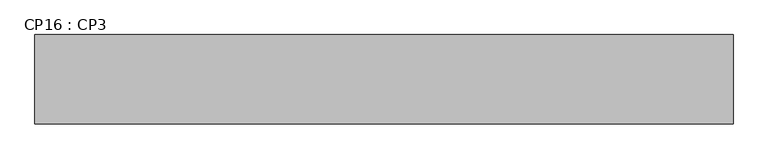
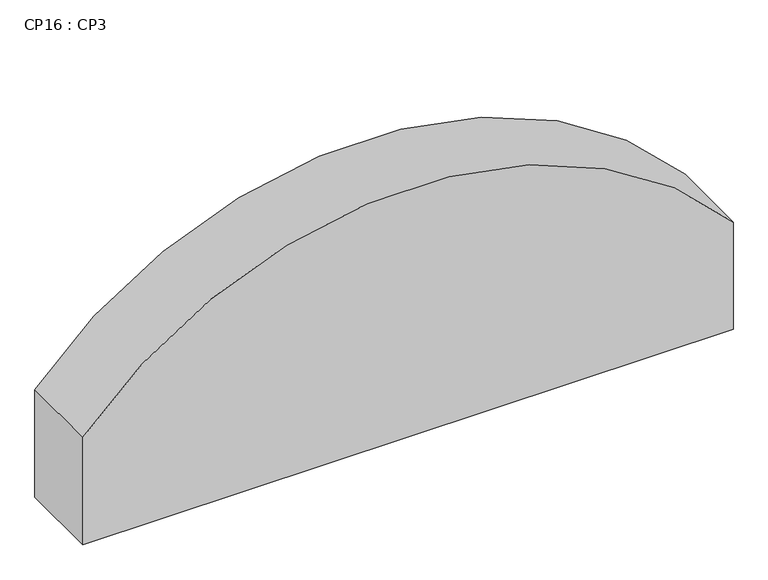
"""IFC4 building model written with IfcOpenShell, lengths in millimetres: beam geometry, CP16 : CP3."""

import ifcopenshell
import ifcopenshell.guid

model = None  # the IFC model being written
_history = None  # IfcOwnerHistory: only IFC2X3 demands one
_inside = {}  # id of a spatial element -> (the spatial element, [elements in it])
_under = {}  # id of a project, library or spatial element -> (it, [spatial elements below it])
_declared = {}  # id of a project -> (the project, [libraries it declares])
_typed = {}  # id of a type object -> (the type object, [elements of that type])
_made_of = {}  # id of a material, layer set ... -> (it, [elements and type objects made of it])


def new_model(schema):
    """Start an empty IFC model of exactly this schema.

    Asked for "IFC4X3", IfcOpenShell would pick the latest addendum, in which some entities
    have other attributes; the version numbers below select the first issue.
    IFC2X3 requires an IfcOwnerHistory on every rooted entity: one is made here for all.
    """
    global model, _history
    if schema == "IFC4X3":
        model = ifcopenshell.file(schema_version=(4, 3, 0, 0))
    else:
        model = ifcopenshell.file(schema=schema)
    _inside.clear()
    _under.clear()
    _declared.clear()
    _typed.clear()
    _made_of.clear()
    _history = None
    if model.schema == "IFC2X3":
        org = make("IfcOrganization", Name="unknown")
        user = make(
            "IfcPersonAndOrganization",
            ThePerson=make("IfcPerson", FamilyName="unknown"),
            TheOrganization=org,
        )
        app = make(
            "IfcApplication",
            ApplicationDeveloper=org,
            Version="unknown",
            ApplicationFullName="unknown",
            ApplicationIdentifier="unknown",
        )
        _history = make(
            "IfcOwnerHistory",
            OwningUser=user,
            OwningApplication=app,
            ChangeAction="ADDED",
            CreationDate=0,
        )
    return model


def make(cls, **values):
    """One entity of the class cls with the attributes given. An attribute that is None is left unset."""
    return model.create_entity(
        cls, **{name: value for name, value in values.items() if value is not None}
    )


def rooted(cls, **values):
    """An entity with a GlobalId (a new one), such as an element, a storey or a relation."""
    return make(cls, GlobalId=ifcopenshell.guid.new(), OwnerHistory=_history, **values)


def si_unit(unit_type, name, prefix=None):
    """IfcSIUnit, for example si_unit("LENGTHUNIT", "METRE", prefix="MILLI")."""
    return make("IfcSIUnit", UnitType=unit_type, Prefix=prefix, Name=name)


def assignment(units):
    """IfcUnitAssignment: the units of a project."""
    return None if units is None else make("IfcUnitAssignment", Units=units)


def point(xyz):
    """IfcCartesianPoint."""
    return None if xyz is None else make("IfcCartesianPoint", Coordinates=xyz)


def direction(xyz):
    """IfcDirection."""
    return None if xyz is None else make("IfcDirection", DirectionRatios=xyz)


def frame(location, z_axis=None, x_axis=None):
    """IfcAxis2Placement3D, a coordinate frame: its origin and axes. An axis left out is left unset."""
    return make(
        "IfcAxis2Placement3D",
        Location=point(location),
        Axis=direction(z_axis),
        RefDirection=direction(x_axis),
    )


def origin():
    """The frame at (0, 0, 0) with its axes left unset."""
    return frame((0.0, 0.0, 0.0))


def place(relative_to, where):
    """IfcLocalPlacement: puts the frame where relative to a parent placement (None: the world)."""
    return make(
        "IfcLocalPlacement", PlacementRelTo=relative_to, RelativePlacement=where
    )


def context(
    kind, dimensions, precision=None, world=None, true_north=None, identifier=None
):
    """IfcGeometricRepresentationContext, for example the 3D "Model" context."""
    return make(
        "IfcGeometricRepresentationContext",
        ContextIdentifier=identifier,
        ContextType=kind,
        CoordinateSpaceDimension=dimensions,
        Precision=precision,
        WorldCoordinateSystem=world,
        TrueNorth=true_north,
    )


def project(units=None, contexts=None):
    """IfcProject with its units and contexts."""
    return rooted(
        "IfcProject",
        Name="project",
        RepresentationContexts=contexts,
        UnitsInContext=assignment(units),
    )


def spatial(cls, under=None, at=None, **own):
    """A site, building, storey or space (cls), placed at a placement, below another one or the project."""
    s = rooted(cls, ObjectPlacement=at, **own)
    if under is not None:
        _under.setdefault(under.id(), (under, []))[1].append(s)
    return s


def circle_curve(where, radius):
    """IfcCircle in the frame where."""
    return make("IfcCircle", Position=where, Radius=radius)


def shape(context_of_items, identifier, shape_type, items):
    """IfcShapeRepresentation: the items that make up one representation, for example the "Body"."""
    return make(
        "IfcShapeRepresentation",
        ContextOfItems=context_of_items,
        RepresentationIdentifier=identifier,
        RepresentationType=shape_type,
        Items=items,
    )


def source(mapping_origin, context_of_items, identifier, shape_type, items):
    """IfcRepresentationMap: a shape defined once, which mapped items show again and again."""
    return make(
        "IfcRepresentationMap",
        MappingOrigin=mapping_origin,
        MappedRepresentation=shape(context_of_items, identifier, shape_type, items),
    )


def transform(
    local_origin,
    x_axis=None,
    y_axis=None,
    z_axis=None,
    scale=None,
    scale2=None,
    scale3=None,
    uniform=True,
):
    """IfcCartesianTransformationOperator3D, or its non-uniform kind. x_axis, y_axis, z_axis: its Axis1, 2, 3."""
    if uniform:
        return make(
            "IfcCartesianTransformationOperator3D",
            Axis1=direction(x_axis),
            Axis2=direction(y_axis),
            LocalOrigin=point(local_origin),
            Scale=scale,
            Axis3=direction(z_axis),
        )
    return make(
        "IfcCartesianTransformationOperator3DnonUniform",
        Axis1=direction(x_axis),
        Axis2=direction(y_axis),
        LocalOrigin=point(local_origin),
        Scale=scale,
        Axis3=direction(z_axis),
        Scale2=scale2,
        Scale3=scale3,
    )


def mapped(mapping_source, mapping_target):
    """IfcMappedItem: shows the shape of a source again, moved by a transform."""
    return make(
        "IfcMappedItem", MappingSource=mapping_source, MappingTarget=mapping_target
    )


def made_of(thing, what):
    """Note that an element or type object is made of a material, layer set ...; save() writes the relation."""
    if what is not None:
        _made_of.setdefault(what.id(), (what, []))[1].append(thing)
    return thing


def element(
    cls,
    number,
    at=None,
    inside=None,
    cuts=None,
    type_object=None,
    material=None,
    context=None,
    identifier="Body",
    shape_type=None,
    held_by="IfcProductDefinitionShape",
    body=None,
    shapes=None,
    **own,
):
    """One element of the class cls, such as IfcWall. Its Tag is "e" and its number.

    at: its placement. inside: the storey or other place that contains it. cuts: it is an
    opening in that element (IfcRelVoidsElement). A single representation is given by context,
    identifier, shape_type and body (its items); several are given by shapes. held_by: the class
    of the entity that holds the representations. save() writes the other relations.
    """
    e = rooted(cls, Tag="e%d" % number, ObjectPlacement=at, **own)
    if body is not None:
        shapes = [shape(context, identifier, shape_type, body)]
    if shapes is not None:
        e.Representation = make(held_by, Representations=shapes)
    if inside is not None:
        _inside.setdefault(inside.id(), (inside, []))[1].append(e)
    if cuts is not None:
        rooted(
            "IfcRelVoidsElement", RelatingBuildingElement=cuts, RelatedOpeningElement=e
        )
    if type_object is not None:
        _typed.setdefault(type_object.id(), (type_object, []))[1].append(e)
    return made_of(e, material)


def aggregate(whole, parts):
    """IfcRelAggregates: a whole, such as a stair, and the parts it consists of."""
    return rooted("IfcRelAggregates", RelatingObject=whole, RelatedObjects=parts)


def save(model, path):
    """Write the relations noted so far, then the file.

    IfcRelAggregates (storeys below a building ...), IfcRelContainedInSpatialStructure (elements
    in a storey), IfcRelDefinesByType, IfcRelAssociatesMaterial and IfcRelDeclares: one each for
    every whole, place, type object, material and project.
    """
    for whole, parts in _under.values():
        aggregate(whole, parts)
    for where, things in _inside.values():
        rooted(
            "IfcRelContainedInSpatialStructure",
            RelatedElements=things,
            RelatingStructure=where,
        )
    for kind, things in _typed.values():
        rooted("IfcRelDefinesByType", RelatedObjects=things, RelatingType=kind)
    for what, things in _made_of.values():
        rooted("IfcRelAssociatesMaterial", RelatedObjects=things, RelatingMaterial=what)
    for by, libraries in _declared.values():
        rooted("IfcRelDeclares", RelatingContext=by, RelatedDefinitions=libraries)
    model.write(path)


def plane_surface(at):
    """IfcPlane: the flat surface through the origin of the frame at, square to its z axis."""
    return make("IfcPlane", Position=at)


def cylinder_surface(at, radius):
    """IfcCylindricalSurface: all points at the distance radius from the z axis of the frame at."""
    return make("IfcCylindricalSurface", Position=at, Radius=radius)


def advanced_brep(points, edges, surfaces, faces):
    """IfcAdvancedBrep: a solid bounded by faces that lie on surfaces and meet in shared edges.

    An edge is (start, end): straight between two places in points (the first is 0);
    or (start, end, curve); or (start, end, curve, False) where it runs against its curve.
    A face is (place in surfaces, loops), or (place, loops, False) where it looks against
    its surface's normal. A loop lists edges by number (the first is 1), with a minus sign
    where the edge is run from its end to its start. The first loop is the outer one.
    """
    corners = [point(p) for p in points]
    vertices = [make("IfcVertexPoint", VertexGeometry=c) for c in corners]
    made = []
    for start, end, *more in edges:
        made.append(
            make(
                "IfcEdgeCurve",
                EdgeStart=vertices[start],
                EdgeEnd=vertices[end],
                EdgeGeometry=more[0] if more else make("IfcPolyline", Points=[corners[start], corners[end]]),
                SameSense=more[1] if len(more) > 1 else True,
            )
        )
    hull = []
    for where, loops, *sense in faces:
        bounds = []
        for j, loop in enumerate(loops):
            ring = [make("IfcOrientedEdge", EdgeElement=made[abs(k) - 1], Orientation=k > 0) for k in loop]
            bounds.append(
                make(
                    "IfcFaceOuterBound" if j == 0 else "IfcFaceBound",
                    Bound=make("IfcEdgeLoop", EdgeList=ring),
                    Orientation=True,
                )
            )
        hull.append(make("IfcAdvancedFace", Bounds=bounds, FaceSurface=surfaces[where], SameSense=sense[0] if sense else True))
    return make("IfcAdvancedBrep", Outer=make("IfcClosedShell", CfsFaces=hull))


def cp16_cp3_4619df2a(model_context):
    return source(origin(), model_context, "Body", "AdvancedBrep", [
        advanced_brep(
        [(10143.2245521, 20099.7448193, 13800.0), (10143.2245521, 20099.7448193, 14620.0), (14843.2245541, 20099.7448193, 14620.0), (14843.2245527, 20099.7448193, 13800.0), (14843.2245541, 19499.6999972, 14620.0), (10143.2245541, 19499.6999972, 14620.0), (10143.2245521, 19499.6999972, 13800.0), (14843.2245527, 19499.6999972, 13800.0)],
        [
            (0, 1),
            (1, 2, circle_curve(frame((12493.2245541, 20099.7448193, 12603.2870371), z_axis=(0.0, 1.0, 0.0), x_axis=(0.0, 0.0, -1.0)), 3096.7129629)),
            (2, 3),
            (3, 0),
            (4, 5, circle_curve(frame((12493.2245541, 19499.6999972, 12603.2870371), z_axis=(0.0, -1.0, 0.0), x_axis=(0.0, 0.0, -1.0)), 3096.7129629)),
            (5, 6),
            (6, 7),
            (7, 4),
            (6, 0),
            (3, 7),
            (4, 2),
            (1, 5),
        ],
        [
            plane_surface(frame((9993.2245542, 20099.7448193, 13800.0), z_axis=(0.0, 1.0, 0.0), x_axis=(0.0, 0.0, 1.0))),
            plane_surface(frame((9993.2245542, 19499.6999972, 13800.0), z_axis=(0.0, -1.0, 0.0), x_axis=(0.0, 0.0, -1.0))),
            plane_surface(frame((14993.2245542, 20099.7448193, 13800.0), z_axis=(0.0, 0.0, -1.0), x_axis=(0.0, -1.0, 0.0))),
            cylinder_surface(frame((12493.2245541, 20099.7448193, 12603.2870371), z_axis=(0.0, 1.0, 0.0), x_axis=(0.0, 0.0, -1.0)), 3096.7129629),
            plane_surface(frame((10143.2245521, 18587.0448193, 14620.0), z_axis=(-1.0, 0.0, 0.0), x_axis=(0.0, -1.0, 0.0))),
            plane_surface(frame((14843.2245527, 18587.0448193, 13800.0), z_axis=(1.0, 0.0, 0.0), x_axis=(0.0, -1.0, 0.0))),
        ],
        [
            (0, [[1, 2, 3, 4]]),
            (1, [[5, 6, 7, 8]]),
            (2, [[9, -4, 10, -7]]),
            (3, [[-5, 11, -2, 12]]),
            (4, [[-1, -9, -6, -12]]),
            (5, [[-3, -11, -8, -10]]),
        ],
    ),
    ])


if __name__ == "__main__":
    model = new_model("IFC4")
    model_context = context("Model", 3, world=origin())
    ifc_project = project(units=[si_unit("LENGTHUNIT", "METRE", prefix="MILLI")], contexts=[model_context])
    site = spatial("IfcSite", under=ifc_project)
    building = spatial("IfcBuilding", under=site)
    placement = place(None, origin())
    cp16_cp3_shape = cp16_cp3_4619df2a(model_context)
    element("IfcBeam", 1, ObjectType="CP16 : CP3", at=placement, inside=building, context=model_context, shape_type="MappedRepresentation", body=[
        mapped(cp16_cp3_shape, transform((0.0, 0.0, 0.0), x_axis=(1.0, 0.0, 0.0), y_axis=(0.0, 1.0, 0.0), z_axis=(0.0, 0.0, 1.0))),
    ])
    save(model, "model.ifc")
